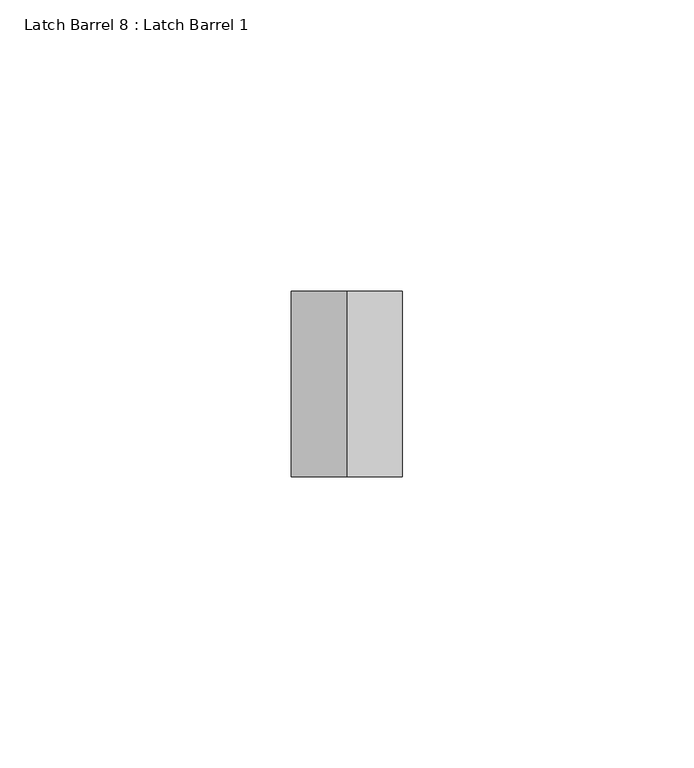
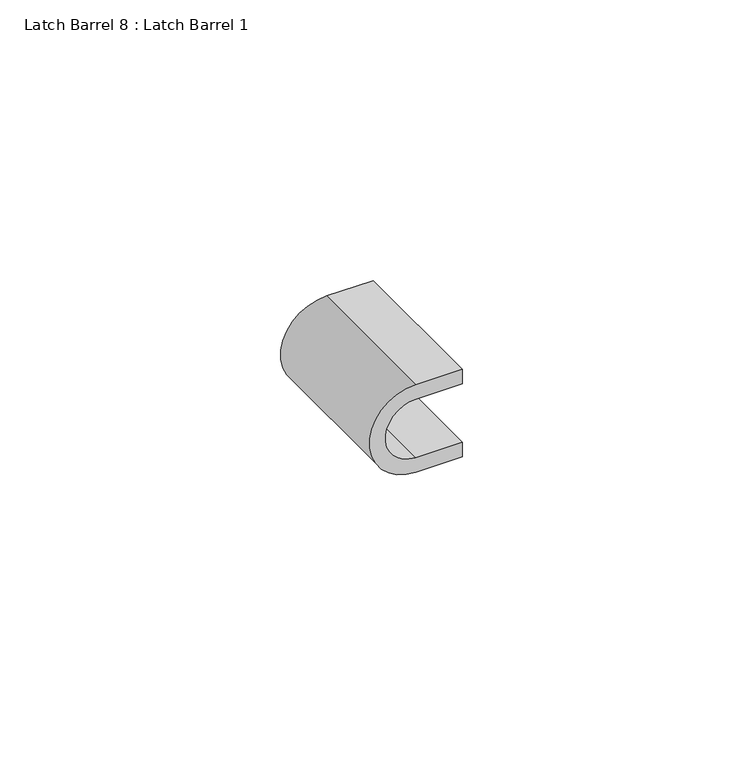
"""IFC4 building model written with IfcOpenShell, lengths in millimetres: proxy geometry, Latch Barrel 8 : Latch Barrel 1."""

from ifc_helpers import new_model, si_unit, point, frame, frame_2d, origin, place, context, project, spatial, polyline, circle_curve, trimmed, segment, composite_curve, outline, extrude, source, transform, mapped, element, save


def latch_barrel_8_latch_barrel_1_0ede4d69(model_context):
    return source(origin(), model_context, "Body", "SweptSolid", [
        extrude(outline(composite_curve([segment(trimmed(circle_curve(frame_2d((1066.8, 587312.7185739)), 6.35), [point((1060.45, 587312.7185739))], [point((1073.15, 587312.7185739))], True, "CARTESIAN"), True, "CONTINUOUS"), segment(polyline([(1073.15, 587312.7185739), (1073.15, 587322.2435739), (1076.325, 587322.2435739), (1076.325, 587312.7185739)]), True, "CONTINUOUS"), segment(trimmed(circle_curve(frame_2d((1066.8, 587312.7185739)), 9.525), [point((1076.325, 587312.7185739))], [point((1057.275, 587312.7185739))], False, "CARTESIAN"), True, "CONTINUOUS"), segment(polyline([(1057.275, 587312.7185739), (1057.275, 587322.2435739), (1060.45, 587322.2435739), (1060.45, 587312.7185739)]), True, "CONTINUOUS")], self_intersect=False)), frame((0.0, -535163.4663841, 0.0), z_axis=(0.0, 1.0, 0.0), x_axis=(0.0, 0.0, 1.0)), (0.0, 0.0, 1.0), 31.75),
    ])


if __name__ == "__main__":
    model = new_model("IFC4")
    model_context = context("Model", 3, world=origin())
    ifc_project = project(units=[si_unit("LENGTHUNIT", "METRE", prefix="MILLI")], contexts=[model_context])
    site = spatial("IfcSite", under=ifc_project)
    building = spatial("IfcBuilding", under=site)
    placement = place(None, origin())
    latch_barrel_8_latch_barrel_1_shape = latch_barrel_8_latch_barrel_1_0ede4d69(model_context)
    element("IfcBuildingElementProxy", 1, Name="Latch Barrel 8 : Latch Barrel 1", ObjectType="Latch Barrel 8 : Latch Barrel 1", at=placement, inside=building, context=model_context, shape_type="MappedRepresentation", body=[
        mapped(latch_barrel_8_latch_barrel_1_shape, transform((0.0, 0.0, 0.0), x_axis=(1.0, 0.0, 0.0), y_axis=(0.0, 1.0, 0.0), z_axis=(0.0, 0.0, 1.0))),
    ])
    save(model, "model.ifc")

# Revit data of these elements
# Element 1 (IfcBuildingElementProxy, "Latch Barrel 8 : Latch Barrel 1")
#   Materials on its faces: "GALV. GATE LATCH"
# Materials
#   "GALV. GATE LATCH": class "Metal", colour RGB 189 187 185, transparency 0, Description = "Carbon steel", Cost = 0
